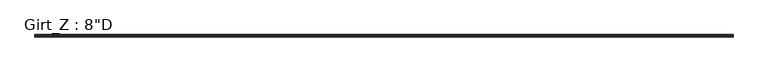
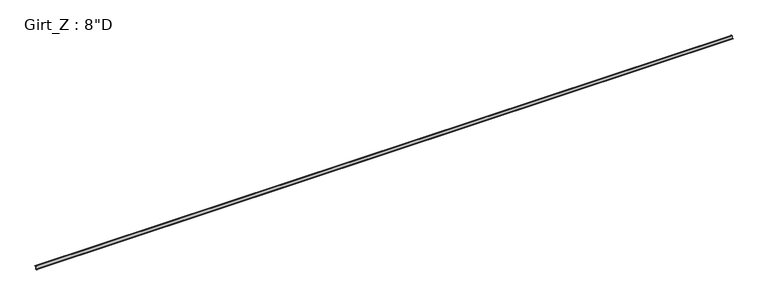
"""IFC4 building model written with IfcOpenShell, lengths in millimetres: beam geometry."""

from ifc_helpers import new_model, si_unit, point, frame, frame_2d, origin, place, context, project, spatial, polyline, circle_curve, trimmed, segment, composite_curve, outline, extrude, source, transform, mapped, element, save


def beam_91b7c892(model_context):
    return source(origin(), model_context, "Body", "SweptSolid", [
        extrude(outline(composite_curve([segment(polyline([(63.5, 101.6), (75.745104, 87.0068534), (73.6169367, 85.221109), (62.204539, 98.821875), (3.3005807, 98.821875)]), True, "CONTINUOUS"), segment(trimmed(circle_curve(frame_2d((3.3741066, 96.8381931)), 1.9850441), [point((3.3005807, 98.821875))], [point((1.3890625, 96.8381931))], True, "CARTESIAN"), True, "CONTINUOUS"), segment(polyline([(1.3890625, 96.8381931), (1.3890625, -96.8375)]), True, "CONTINUOUS"), segment(trimmed(circle_curve(frame_2d((-3.3734375, -96.8375)), 4.7625), [point((1.3890625, -96.8375))], [point((-3.3734375, -101.6))], False, "CARTESIAN"), True, "CONTINUOUS"), segment(polyline([(-3.3734375, -101.6), (-63.5, -101.6), (-75.745104, -87.0068534), (-73.6169367, -85.221109), (-62.204539, -98.821875), (-3.2694106, -98.821875)]), True, "CONTINUOUS"), segment(trimmed(circle_curve(frame_2d((-3.3748024, -96.8389339)), 1.9857399), [point((-3.2694106, -98.821875))], [point((-1.3890625, -96.8389339))], True, "CARTESIAN"), True, "CONTINUOUS"), segment(polyline([(-1.3890625, -96.8389339), (-1.3890625, 96.8375)]), True, "CONTINUOUS"), segment(trimmed(circle_curve(frame_2d((3.3734375, 96.8375)), 4.7625), [point((-1.3890625, 96.8375))], [point((3.3734375, 101.6))], False, "CARTESIAN"), True, "CONTINUOUS"), segment(polyline([(3.3734375, 101.6), (63.5, 101.6)]), True, "CONTINUOUS")], self_intersect=False)), frame((-23999.825, 0.0, 0.0), z_axis=(1.0, 0.0, 0.0), x_axis=(0.0, 1.0, 0.0)), (0.0, 0.0, 1.0), 47844.075),
    ])


if __name__ == "__main__":
    model = new_model("IFC4")
    model_context = context("Model", 3, world=origin())
    ifc_project = project(units=[si_unit("LENGTHUNIT", "METRE", prefix="MILLI")], contexts=[model_context])
    site = spatial("IfcSite", under=ifc_project)
    building = spatial("IfcBuilding", under=site)
    placement = place(None, origin())
    beam_shape = beam_91b7c892(model_context)
    element("IfcBeam", 1, ObjectType="Girt_Z : 8\"D", at=placement, inside=building, context=model_context, shape_type="MappedRepresentation", body=[
        mapped(beam_shape, transform((0.0, 0.0, 0.0), x_axis=(1.0, 0.0, 0.0), y_axis=(0.0, 1.0, 0.0), z_axis=(0.0, 0.0, 1.0))),
    ])
    save(model, "model.ifc")

# Revit data of these elements
# Type "Girt_Z : 8\"D"
#   Web_Thickness = 0' - 0 7/64"
#   Length [instance default] = 10' - 0"
#   Leg_1 = 0' - 2 1/2"
#   Height = 0' - 8"
#   Structural Material [instance default] = none
